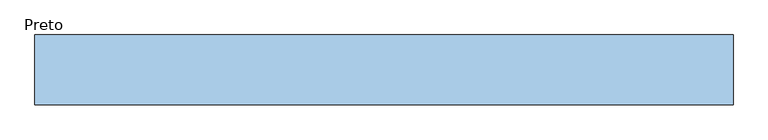
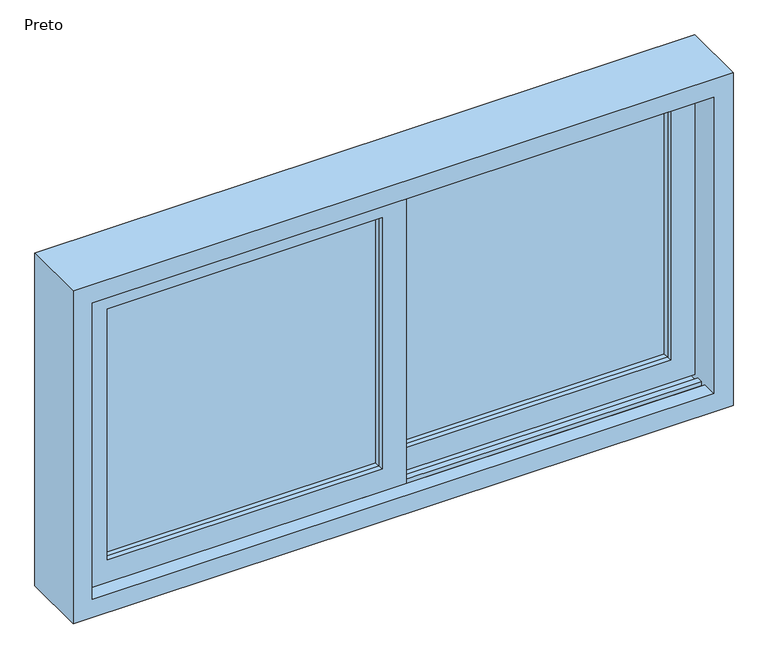
"""IFC4 building model written with IfcOpenShell, lengths in millimetres: window geometry, Blks_Cons Weiku_Janela de Correr 02 Folhas : Preto."""

from ifc_helpers import new_model, si_unit, frame, origin, place, context, project, spatial, polyline, outline, extrude, faceted_brep, source, transform, mapped, element, save


def preto_280b240e(model_context):
    return source(origin(), model_context, "Body", "SolidModel", [
        faceted_brep([(27.0, 13.0, 898.0), (27.0, 13.0, 1502.0), (27.0, 18.0, 1502.0), (27.0, 18.0, 898.0), (32.0, 18.0, 903.0), (32.0, 18.0, 1497.0), (652.0, 13.0, 1502.0), (652.0, 18.0, 1502.0), (647.0, 18.0, 1497.0), (652.0, 13.0, 898.0), (652.0, 18.0, 898.0), (647.0, 18.0, 903.0)], [[[0, 1, 2, 3]], [[4, 5, 1, 0]], [[1, 6, 7, 2]], [[5, 8, 6, 1]], [[6, 9, 10, 7]], [[8, 11, 9, 6]], [[3, 2, 7, 10], [5, 4, 11, 8]], [[9, 0, 3, 10]], [[11, 4, 0, 9]]]),
        faceted_brep([(652.0, 27.0, 898.0), (652.0, 27.0, 1502.0), (652.0, 22.0, 1502.0), (652.0, 22.0, 898.0), (27.0, 27.0, 1502.0), (27.0, 22.0, 1502.0), (27.0, 27.0, 898.0), (27.0, 22.0, 898.0), (647.0, 22.0, 1497.0), (647.0, 22.0, 903.0), (32.0, 22.0, 903.0), (32.0, 22.0, 1497.0)], [[[0, 1, 2, 3]], [[1, 4, 5, 2]], [[4, 6, 7, 5]], [[3, 2, 5, 7], [8, 9, 10, 11]], [[6, 0, 3, 7]], [[9, 8, 1, 0]], [[8, 11, 4, 1]], [[11, 10, 6, 4]], [[10, 9, 0, 6]]]),
        extrude(outline(polyline([(652.0, 22.0), (652.0, 18.0), (27.0, 18.0), (27.0, 22.0), (652.0, 22.0)])), frame((0.0, 0.0, 898.0), z_axis=(0.0, 0.0, 1.0), x_axis=(1.0, 0.0, 0.0)), (0.0, 0.0, 1.0), 604.0),
        extrude(outline(polyline([(844.0, 706.0), (1556.0, 706.0), (1556.0, -27.0), (844.0, -27.0), (844.0, 706.0)]), holes=[polyline([(1502.0, 27.0), (1502.0, 652.0), (898.0, 652.0), (898.0, 27.0), (1502.0, 27.0)])]), frame((0.0, 0.0, 0.0), z_axis=(0.0, 1.0, 0.0), x_axis=(0.0, 0.0, 1.0)), (0.0, 0.0, 1.0), 40.0),
        faceted_brep([(-652.0, -27.0, 898.0), (-652.0, -27.0, 1502.0), (-652.0, -22.0, 1502.0), (-652.0, -22.0, 898.0), (-647.0, -22.0, 903.0), (-647.0, -22.0, 1497.0), (-27.0, -27.0, 1502.0), (-27.0, -22.0, 1502.0), (-32.0, -22.0, 1497.0), (-27.0, -27.0, 898.0), (-27.0, -22.0, 898.0), (-32.0, -22.0, 903.0)], [[[0, 1, 2, 3]], [[4, 5, 1, 0]], [[1, 6, 7, 2]], [[5, 8, 6, 1]], [[6, 9, 10, 7]], [[8, 11, 9, 6]], [[3, 2, 7, 10], [5, 4, 11, 8]], [[9, 0, 3, 10]], [[11, 4, 0, 9]]]),
        faceted_brep([(-27.0, -13.0, 898.0), (-27.0, -13.0, 1502.0), (-27.0, -18.0, 1502.0), (-27.0, -18.0, 898.0), (-652.0, -13.0, 1502.0), (-652.0, -18.0, 1502.0), (-652.0, -13.0, 898.0), (-652.0, -18.0, 898.0), (-32.0, -18.0, 1497.0), (-32.0, -18.0, 903.0), (-647.0, -18.0, 903.0), (-647.0, -18.0, 1497.0)], [[[0, 1, 2, 3]], [[1, 4, 5, 2]], [[4, 6, 7, 5]], [[3, 2, 5, 7], [8, 9, 10, 11]], [[6, 0, 3, 7]], [[9, 8, 1, 0]], [[8, 11, 4, 1]], [[11, 10, 6, 4]], [[10, 9, 0, 6]]]),
        extrude(outline(polyline([(-27.0, -18.0), (-27.0, -22.0), (-652.0, -22.0), (-652.0, -18.0), (-27.0, -18.0)])), frame((0.0, 0.0, 898.0), z_axis=(0.0, 0.0, 1.0), x_axis=(1.0, 0.0, 0.0)), (0.0, 0.0, 1.0), 604.0),
        extrude(outline(polyline([(844.0, 27.0), (1556.0, 27.0), (1556.0, -706.0), (844.0, -706.0), (844.0, 27.0)]), holes=[polyline([(1502.0, -652.0), (1502.0, -27.0), (898.0, -27.0), (898.0, -652.0), (1502.0, -652.0)])]), frame((0.0, -40.0, 0.0), z_axis=(0.0, 1.0, 0.0), x_axis=(0.0, 0.0, 1.0)), (0.0, 0.0, 1.0), 40.0),
        faceted_brep([(706.0, -75.0, 844.0), (706.0, -40.0, 844.0), (-706.0, -40.0, 844.0), (-706.0, -75.0, 844.0), (-706.0, 75.0, 844.0), (-706.0, 40.0, 844.0), (706.0, 40.0, 844.0), (706.0, 75.0, 844.0), (-706.0, 13.0, 844.0), (706.0, 13.0, 844.0), (706.0, 27.0, 844.0), (-706.0, 27.0, 844.0), (-706.0, -27.0, 844.0), (706.0, -27.0, 844.0), (706.0, -13.0, 844.0), (-706.0, -13.0, 844.0), (750.0, -75.0, 800.0), (750.0, -75.0, 1600.0), (-750.0, -75.0, 1600.0), (-750.0, -75.0, 800.0), (-706.0, -75.0, 1556.0), (706.0, -75.0, 1556.0), (-706.0, -40.0, 834.0), (-706.0, -27.0, 834.0), (-706.0, -13.0, 834.0), (-706.0, 13.0, 834.0), (-706.0, 27.0, 834.0), (-706.0, 40.0, 834.0), (-706.0, 75.0, 1556.0), (-706.0, 40.0, 1556.0), (-706.0, 40.0, 1566.0), (-706.0, 27.0, 1566.0), (-706.0, 27.0, 1556.0), (-706.0, 13.0, 1556.0), (-706.0, 13.0, 1566.0), (-706.0, -13.0, 1566.0), (-706.0, -13.0, 1556.0), (-706.0, -27.0, 1556.0), (-706.0, -27.0, 1566.0), (-706.0, -40.0, 1566.0), (-706.0, -40.0, 1556.0), (706.0, -40.0, 834.0), (706.0, -40.0, 1556.0), (706.0, -40.0, 1566.0), (706.0, -27.0, 1566.0), (706.0, -27.0, 1556.0), (706.0, -13.0, 1556.0), (706.0, -13.0, 1566.0), (706.0, 13.0, 1566.0), (706.0, 13.0, 1556.0), (706.0, 27.0, 1556.0), (706.0, 27.0, 1566.0), (706.0, 40.0, 1566.0), (706.0, 40.0, 1556.0), (706.0, 75.0, 1556.0), (706.0, 40.0, 834.0), (706.0, 27.0, 834.0), (706.0, 13.0, 834.0), (706.0, -13.0, 834.0), (706.0, -27.0, 834.0), (-750.0, 75.0, 800.0), (-750.0, 75.0, 1600.0), (750.0, 75.0, 1600.0), (750.0, 75.0, 800.0)], [[[0, 1, 2, 3]], [[4, 5, 6, 7]], [[8, 9, 10, 11]], [[12, 13, 14, 15]], [[16, 17, 18, 19], [3, 20, 21, 0]], [[3, 2, 22, 23, 12, 15, 24, 25, 8, 11, 26, 27, 5, 4, 28, 29, 30, 31, 32, 33, 34, 35, 36, 37, 38, 39, 40, 20]], [[22, 2, 1, 41]], [[21, 42, 43, 44, 45, 46, 47, 48, 49, 50, 51, 52, 53, 54, 7, 6, 55, 56, 10, 9, 57, 58, 14, 13, 59, 41, 1, 0]], [[60, 61, 62, 63], [7, 54, 28, 4]], [[55, 6, 5, 27]], [[56, 26, 11, 10]], [[9, 8, 25, 57]], [[58, 24, 15, 14]], [[13, 12, 23, 59]], [[63, 62, 17, 16]], [[16, 19, 60, 63]], [[19, 18, 61, 60]], [[55, 27, 26, 56]], [[57, 25, 24, 58]], [[59, 23, 22, 41]], [[20, 40, 42, 21]], [[54, 53, 29, 28]], [[32, 50, 49, 33]], [[36, 46, 45, 37]], [[18, 17, 62, 61]], [[46, 36, 35, 47]], [[47, 35, 34, 48]], [[48, 34, 33, 49]], [[50, 32, 31, 51]], [[51, 31, 30, 52]], [[30, 29, 53, 52]], [[43, 42, 40, 39]], [[43, 39, 38, 44]], [[44, 38, 37, 45]]]),
    ])


if __name__ == "__main__":
    model = new_model("IFC4")
    model_context = context("Model", 3, world=origin())
    ifc_project = project(units=[si_unit("LENGTHUNIT", "METRE", prefix="MILLI")], contexts=[model_context])
    site = spatial("IfcSite", under=ifc_project)
    building = spatial("IfcBuilding", under=site)
    placement = place(None, origin())
    preto_shape = preto_280b240e(model_context)
    element("IfcWindow", 1, ObjectType="Blks_Cons Weiku_Janela de Correr 02 Folhas : Preto", at=placement, inside=building, context=model_context, shape_type="MappedRepresentation", body=[
        mapped(preto_shape, transform((0.0, 0.0, 0.0), x_axis=(1.0, 0.0, 0.0), y_axis=(0.0, 1.0, 0.0), z_axis=(0.0, 0.0, 1.0))),
    ])
    save(model, "model.ifc")

# Revit data of these elements
# Type "Blks_Cons Weiku_Janela de Correr 02 Folhas : Preto"
#   Type Mark = "J26"
#   Type Comments = "Janela de Correr 02 Folhas"
#   Manufacturer = "Weiku"
#   Created By / Criado Por / Creado por = "Blocks"
#   Author URL = "https://BlocksRvt.com/"
#   Author Contact = "info@blocksrvt.com"
#   Assembly Code = "Cons"
#   c [instance default] = 250 mm
#   b [instance default] = 912 mm
#   a [instance default] = 983 mm
#   Rough Width [instance default] = 2000 mm
#   Width [instance default] = 1912 mm
#   Espessura Folha [instance default] = 40 mm
#   Rough Height [instance default] = 1000 mm
#   Height [instance default] = 912 mm
#   Abertura Janela Equerda [instance default] = 0 mm
#   Abertura Janela Direita [instance default] = 0 mm
#   Vidro = .vidro_growarq
#   Vedação = Blks - Rubber - Black
#   Janela = Blks - Plastic - Black - Glazed
#   Wall Closure = (empty or 0)
# Element 1 (IfcWindow, "Blks_Cons Weiku_Janela de Correr 02 Folhas : Preto")
#   b = 712 mm
#   a = 733 mm
#   Rough Width = 1500 mm
#   Width = 1412 mm
#   Rough Height = 800 mm
#   Height = 712 mm
#   Materials on its faces: "Blks - Plastic - Black - Glazed", "Blks - Rubber - Black", ".vidro_growarq"
# Materials
#   ".vidro_growarq": class "Vidro", colour RGB 200 215 215, transparency 0.6, Description = "Vidroverde", Cost = 0
#   "Blks - Rubber - Black": class "Paint/Coating", colour RGB 38 38 38, transparency 0, Cost = 0
#   "Blks - Plastic - Black - Glazed": class "Plastic", colour RGB 25 25 25, transparency 0, Cost = 0
